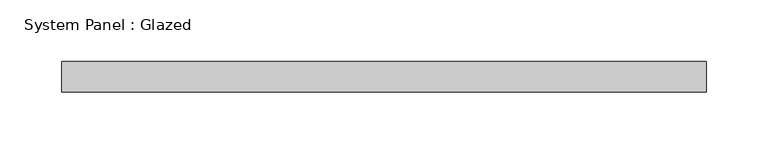
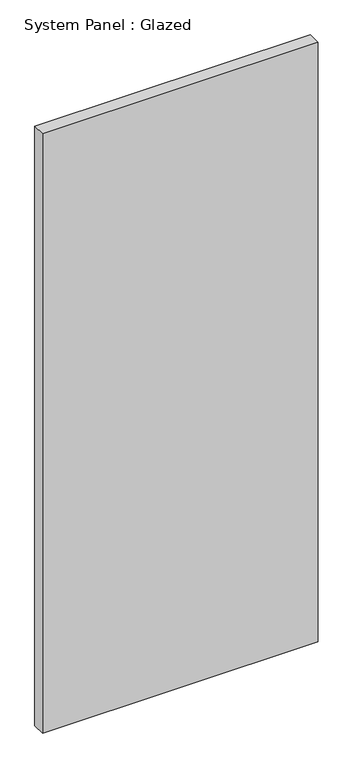
"""IFC4 building model written with IfcOpenShell, lengths in millimetres: plate geometry, System Panel : Glazed."""

from ifc_helpers import new_model, si_unit, origin, origin_with_axes, place, context, project, spatial, polyline, outline, extrude, source, transform, mapped, element, save


def system_panel_glazed_5241e6d5(model_context):
    return source(origin(), model_context, "Body", "SweptSolid", [
        extrude(outline(polyline([(261.3636364, 24.5), (-261.3636364, 24.5), (-261.3636364, 49.5), (261.3636364, 49.5), (261.3636364, 24.5)])), origin_with_axes(), (0.0, 0.0, 1.0), 1200.0),
    ])


if __name__ == "__main__":
    model = new_model("IFC4")
    model_context = context("Model", 3, world=origin())
    ifc_project = project(units=[si_unit("LENGTHUNIT", "METRE", prefix="MILLI")], contexts=[model_context])
    site = spatial("IfcSite", under=ifc_project)
    building = spatial("IfcBuilding", under=site)
    placement = place(None, origin())
    system_panel_glazed_shape = system_panel_glazed_5241e6d5(model_context)
    element("IfcPlate", 1, ObjectType="System Panel : Glazed", at=placement, inside=building, context=model_context, shape_type="MappedRepresentation", body=[
        mapped(system_panel_glazed_shape, transform((0.0, 0.0, 0.0), x_axis=(1.0, 0.0, 0.0), y_axis=(0.0, 1.0, 0.0), z_axis=(0.0, 0.0, 1.0))),
    ])
    save(model, "model.ifc")

# Revit data of these elements
# Element 1 (IfcPlate, "System Panel : Glazed")
#   Materials on its faces: "Glass"
# Materials
#   "Glass": class "Glass", colour RGB 218 227 224, transparency 0.85, Description = "Soda Lime Glass", Cost = 0
